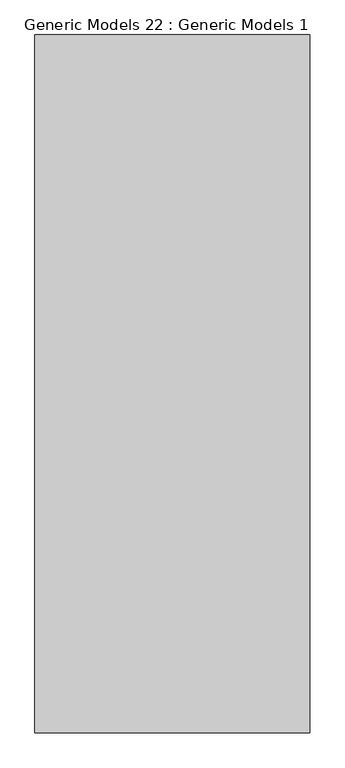
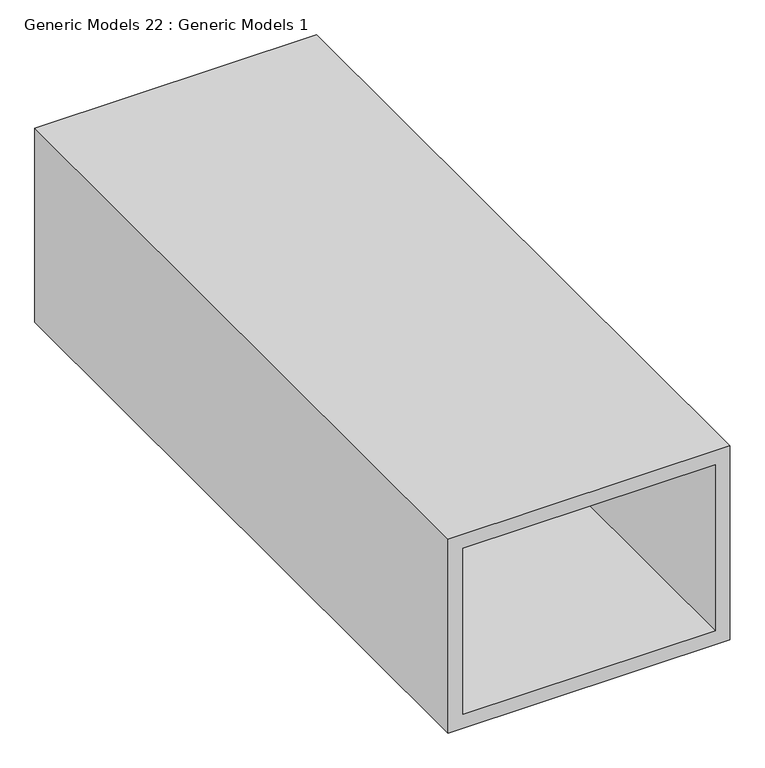
"""IFC4 building model written with IfcOpenShell, lengths in millimetres: proxy geometry, Generic Models 22 : Generic Models 1."""

from ifc_helpers import new_model, si_unit, frame, origin, place, context, project, spatial, polyline, outline, extrude, source, transform, mapped, element, save


def generic_models_22_generic_models_1_b0009ec1(model_context):
    return source(origin(), model_context, "Body", "SweptSolid", [
        extrude(outline(polyline([(2381.25, 51148.3797769), (2381.25, 50668.1069345), (2032.0, 50668.1069345), (2032.0, 51148.3797769), (2381.25, 51148.3797769)]), holes=[polyline([(2355.85, 51122.9797769), (2057.4, 51122.9797769), (2057.4, 50693.5069345), (2355.85, 50693.5069345), (2355.85, 51122.9797769)])]), frame((0.0, 0.0, 0.0), z_axis=(0.0, 1.0, 0.0), x_axis=(0.0, 0.0, 1.0)), (0.0, 0.0, 1.0), 1219.2),
    ])


if __name__ == "__main__":
    model = new_model("IFC4")
    model_context = context("Model", 3, world=origin())
    ifc_project = project(units=[si_unit("LENGTHUNIT", "METRE", prefix="MILLI")], contexts=[model_context])
    site = spatial("IfcSite", under=ifc_project)
    building = spatial("IfcBuilding", under=site)
    placement = place(None, origin())
    generic_models_22_generic_models_1_shape = generic_models_22_generic_models_1_b0009ec1(model_context)
    element("IfcBuildingElementProxy", 1, Name="Generic Models 22 : Generic Models 1", ObjectType="Generic Models 22 : Generic Models 1", at=placement, inside=building, context=model_context, shape_type="MappedRepresentation", body=[
        mapped(generic_models_22_generic_models_1_shape, transform((0.0, 0.0, 0.0), x_axis=(1.0, 0.0, 0.0), y_axis=(0.0, 1.0, 0.0), z_axis=(0.0, 0.0, 1.0))),
    ])
    save(model, "model.ifc")

# Revit data of these elements
# Element 1 (IfcBuildingElementProxy, "Generic Models 22 : Generic Models 1")
#   Materials on its faces: "IF THERE'S AN OPEN AIR WAY PATH, THROUGH THE DUCTS, FROM ONE ROOM TO THE OTHER, EITHER 1)LINE THE INTERIOR OF THE DUCT W/ SOUNDABSORPTIVE MATERIAL AND/OR 2) USE A 'DUCT BAFFLE BOX' TO MUFFLE THE MIGRATING SOUND"
# Materials
#   "IF THERE'S AN OPEN AIR WAY PATH, THROUGH THE DUCTS, FROM ONE ROOM TO THE OTHER, EITHER 1)LINE THE INTERIOR OF THE DUCT W/ SOUNDABSORPTIVE MATERIAL AND/OR 2) USE A 'DUCT BAFFLE BOX' TO MUFFLE THE MIGRATING SOUND": class "Generic", colour RGB 127 127 127, transparency 0, Description = "Rigid foam insulation board", Cost = 0
